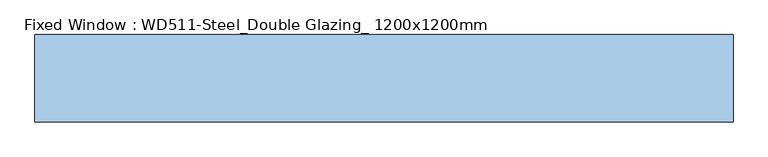
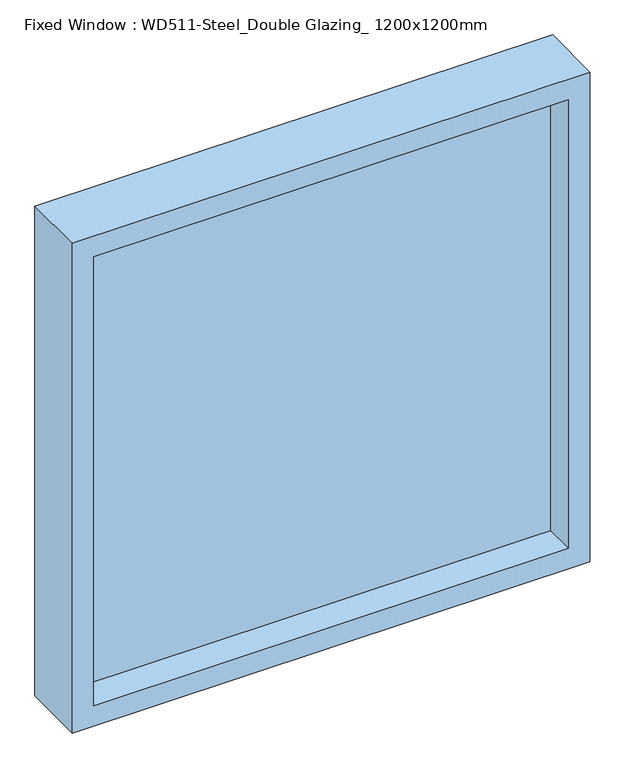
"""IFC4 building model written with IfcOpenShell, lengths in millimetres: window geometry, Fixed Window : WD511-Steel_Double Glazing_ 1200x1200mm."""

from ifc_helpers import new_model, si_unit, frame, origin, place, context, project, spatial, polyline, outline, extrude, source, transform, mapped, element, save


def fixed_window_wd511_steel_double_glazing_1200x1200mm_53d069df(model_context):
    return source(origin(), model_context, "Body", "SweptSolid", [
        extrude(outline(polyline([(-550.0, 3.0), (550.0, 3.0), (550.0, -3.0), (-550.0, -3.0), (-550.0, 3.0)])), frame((0.0, 0.0, 850.0), z_axis=(0.0, 0.0, 1.0), x_axis=(1.0, 0.0, 0.0)), (0.0, 0.0, 1.0), 1100.0),
        extrude(outline(polyline([(2000.0, -600.0), (800.0, -600.0), (800.0, 600.0), (2000.0, 600.0), (2000.0, -600.0)]), holes=[polyline([(1950.0, -550.0), (1950.0, 550.0), (850.0, 550.0), (850.0, -550.0), (1950.0, -550.0)])]), frame((0.0, -75.0, 0.0), z_axis=(0.0, 1.0, 0.0), x_axis=(0.0, 0.0, 1.0)), (0.0, 0.0, 1.0), 150.0),
    ])


if __name__ == "__main__":
    model = new_model("IFC4")
    model_context = context("Model", 3, world=origin())
    ifc_project = project(units=[si_unit("LENGTHUNIT", "METRE", prefix="MILLI")], contexts=[model_context])
    site = spatial("IfcSite", under=ifc_project)
    building = spatial("IfcBuilding", under=site)
    placement = place(None, origin())
    fixed_window_wd511_steel_double_glazing_1200x1200mm_shape = fixed_window_wd511_steel_double_glazing_1200x1200mm_53d069df(model_context)
    element("IfcWindow", 1, ObjectType="Fixed Window : WD511-Steel_Double Glazing_ 1200x1200mm", at=placement, inside=building, context=model_context, shape_type="MappedRepresentation", body=[
        mapped(fixed_window_wd511_steel_double_glazing_1200x1200mm_shape, transform((0.0, 0.0, 0.0), x_axis=(1.0, 0.0, 0.0), y_axis=(0.0, 1.0, 0.0), z_axis=(0.0, 0.0, 1.0))),
    ])
    save(model, "model.ifc")

# Revit data of these elements
# Type "Fixed Window : WD511-Steel_Double Glazing_ 1200x1200mm"
#   Description = "Steel Frame + 2 x T=6mm + T12mm Air Space"
#   Type Mark = ""
#   Analytic Construction = "<None>"
#   창 두께 = 150 mm
#   Height = 1200 mm
#   절반 창 두께 = 75 mm
#   기본 씰 높이 = 800 mm
#   Width = 1200 mm
#   Define Thermal Properties by = 1
#   창 패널 = AW2 창 패널
#   창 프레임 = A04AQ126-00002_Steel Window_None FP
#   Wall Closure = (empty or 0)
# Element 1 (IfcWindow, "Fixed Window : WD511-Steel_Double Glazing_ 1200x1200mm")
#   Materials on its faces: "A04AQ126-00002_Steel Window_None FP", "AW2 창 패널"
# Materials
#   "AW2 창 패널": class "유리", colour RGB 0 0 255, transparency 0.75
#   "A04AQ126-00002_Steel Window_None FP": class "금속", colour RGB 247 247 247, transparency 0, W00) Work Master Code = "A04AQ126-00002", W01) Work Master_Lv1 = "Finishing Work", W02) Work Master_Lv2 = "Door & Window Work", W03) Work Master_Spec.1 = "Steel Window", W04) Work Master_Spec.2 = "Fire Protective Rating: N/A", W05) Work Master_Spec.3 = "w/ Hardware & Accessories", Cost = 0
